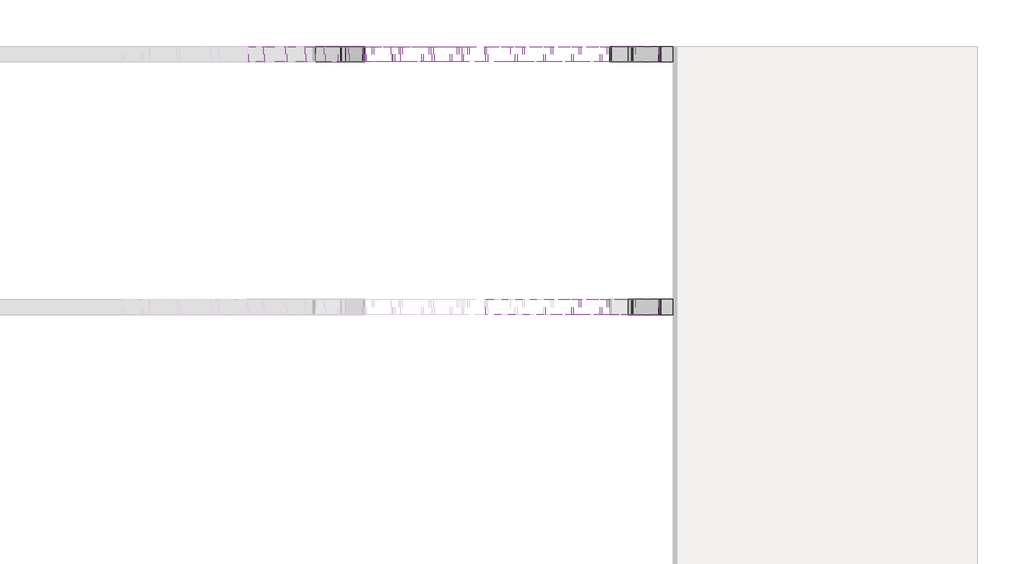
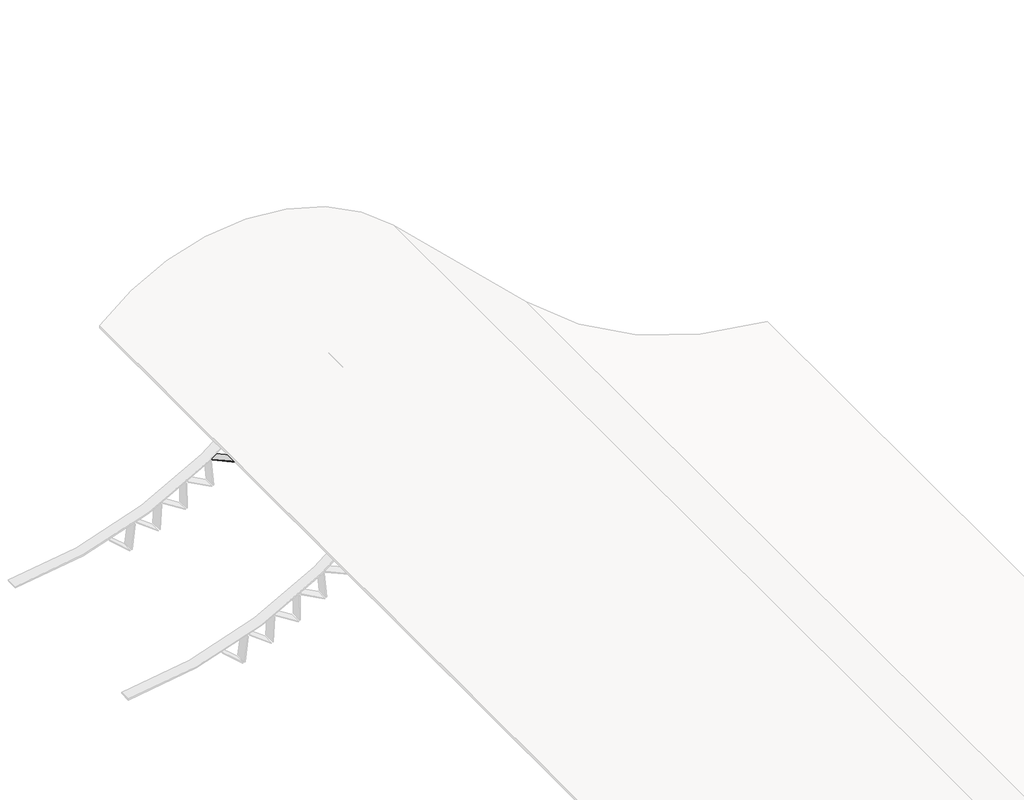
# One storey, part 16 of 16: 78 beams.
"""IFC4 building model written with IfcOpenShell, lengths in millimetres."""

import ifcopenshell
import ifcopenshell.guid

model = None  # the IFC model being written
_history = None  # IfcOwnerHistory: only IFC2X3 demands one
_inside = {}  # id of a spatial element -> (the spatial element, [elements in it])
_under = {}  # id of a project, library or spatial element -> (it, [spatial elements below it])
_declared = {}  # id of a project -> (the project, [libraries it declares])
_typed = {}  # id of a type object -> (the type object, [elements of that type])
_made_of = {}  # id of a material, layer set ... -> (it, [elements and type objects made of it])


def new_model(schema):
    """Start an empty IFC model of exactly this schema.

    Asked for "IFC4X3", IfcOpenShell would pick the latest addendum, in which some entities
    have other attributes; the version numbers below select the first issue.
    IFC2X3 requires an IfcOwnerHistory on every rooted entity: one is made here for all.
    """
    global model, _history
    if schema == "IFC4X3":
        model = ifcopenshell.file(schema_version=(4, 3, 0, 0))
    else:
        model = ifcopenshell.file(schema=schema)
    _inside.clear()
    _under.clear()
    _declared.clear()
    _typed.clear()
    _made_of.clear()
    _history = None
    if model.schema == "IFC2X3":
        org = make("IfcOrganization", Name="unknown")
        user = make(
            "IfcPersonAndOrganization",
            ThePerson=make("IfcPerson", FamilyName="unknown"),
            TheOrganization=org,
        )
        app = make(
            "IfcApplication",
            ApplicationDeveloper=org,
            Version="unknown",
            ApplicationFullName="unknown",
            ApplicationIdentifier="unknown",
        )
        _history = make(
            "IfcOwnerHistory",
            OwningUser=user,
            OwningApplication=app,
            ChangeAction="ADDED",
            CreationDate=0,
        )
    return model


def make(cls, **values):
    """One entity of the class cls with the attributes given. An attribute that is None is left unset."""
    return model.create_entity(
        cls, **{name: value for name, value in values.items() if value is not None}
    )


def rooted(cls, **values):
    """An entity with a GlobalId (a new one), such as an element, a storey or a relation."""
    return make(cls, GlobalId=ifcopenshell.guid.new(), OwnerHistory=_history, **values)


def si_unit(unit_type, name, prefix=None):
    """IfcSIUnit, for example si_unit("LENGTHUNIT", "METRE", prefix="MILLI")."""
    return make("IfcSIUnit", UnitType=unit_type, Prefix=prefix, Name=name)


def assignment(units):
    """IfcUnitAssignment: the units of a project."""
    return None if units is None else make("IfcUnitAssignment", Units=units)


def point(xyz):
    """IfcCartesianPoint."""
    return None if xyz is None else make("IfcCartesianPoint", Coordinates=xyz)


def direction(xyz):
    """IfcDirection."""
    return None if xyz is None else make("IfcDirection", DirectionRatios=xyz)


def frame(location, z_axis=None, x_axis=None):
    """IfcAxis2Placement3D, a coordinate frame: its origin and axes. An axis left out is left unset."""
    return make(
        "IfcAxis2Placement3D",
        Location=point(location),
        Axis=direction(z_axis),
        RefDirection=direction(x_axis),
    )


def frame_2d(location, x_axis=None):
    """IfcAxis2Placement2D, a coordinate frame in the plane: its origin and x axis."""
    return make(
        "IfcAxis2Placement2D", Location=point(location), RefDirection=direction(x_axis)
    )


def origin():
    """The frame at (0, 0, 0) with its axes left unset."""
    return frame((0.0, 0.0, 0.0))


def place(relative_to, where):
    """IfcLocalPlacement: puts the frame where relative to a parent placement (None: the world)."""
    return make(
        "IfcLocalPlacement", PlacementRelTo=relative_to, RelativePlacement=where
    )


def context(
    kind, dimensions, precision=None, world=None, true_north=None, identifier=None
):
    """IfcGeometricRepresentationContext, for example the 3D "Model" context."""
    return make(
        "IfcGeometricRepresentationContext",
        ContextIdentifier=identifier,
        ContextType=kind,
        CoordinateSpaceDimension=dimensions,
        Precision=precision,
        WorldCoordinateSystem=world,
        TrueNorth=true_north,
    )


def project(units=None, contexts=None):
    """IfcProject with its units and contexts."""
    return rooted(
        "IfcProject",
        Name="project",
        RepresentationContexts=contexts,
        UnitsInContext=assignment(units),
    )


def spatial(cls, under=None, at=None, **own):
    """A site, building, storey or space (cls), placed at a placement, below another one or the project."""
    s = rooted(cls, ObjectPlacement=at, **own)
    if under is not None:
        _under.setdefault(under.id(), (under, []))[1].append(s)
    return s


def polyline(points):
    """IfcPolyline through the points."""
    return make("IfcPolyline", Points=[point(p) for p in points])


def circle_curve(where, radius):
    """IfcCircle in the frame where."""
    return make("IfcCircle", Position=where, Radius=radius)


def trimmed(basis, trim1, trim2, sense, master):
    """IfcTrimmedCurve: the piece of a basis curve between two trims."""
    return make(
        "IfcTrimmedCurve",
        BasisCurve=basis,
        Trim1=trim1,
        Trim2=trim2,
        SenseAgreement=sense,
        MasterRepresentation=master,
    )


def segment(curve, same_sense, transition):
    """IfcCompositeCurveSegment."""
    return make(
        "IfcCompositeCurveSegment",
        Transition=transition,
        SameSense=same_sense,
        ParentCurve=curve,
    )


def composite_curve(segments, self_intersect=None):
    """IfcCompositeCurve: segments joined end to end."""
    return make("IfcCompositeCurve", Segments=segments, SelfIntersect=self_intersect)


def outline(outer, holes=None, kind="AREA"):
    """IfcArbitraryClosedProfileDef: a profile drawn as a closed curve; with holes, ...WithVoids."""
    if holes is None:
        return make("IfcArbitraryClosedProfileDef", ProfileType=kind, OuterCurve=outer)
    return make(
        "IfcArbitraryProfileDefWithVoids",
        ProfileType=kind,
        OuterCurve=outer,
        InnerCurves=holes,
    )


def extrude(swept, where, along, depth):
    """IfcExtrudedAreaSolid: the profile swept, set in the frame where, extruded along a direction by depth."""
    return make(
        "IfcExtrudedAreaSolid",
        SweptArea=swept,
        Position=where,
        ExtrudedDirection=direction(along),
        Depth=depth,
    )


def shape(context_of_items, identifier, shape_type, items):
    """IfcShapeRepresentation: the items that make up one representation, for example the "Body"."""
    return make(
        "IfcShapeRepresentation",
        ContextOfItems=context_of_items,
        RepresentationIdentifier=identifier,
        RepresentationType=shape_type,
        Items=items,
    )


def source(mapping_origin, context_of_items, identifier, shape_type, items):
    """IfcRepresentationMap: a shape defined once, which mapped items show again and again."""
    return make(
        "IfcRepresentationMap",
        MappingOrigin=mapping_origin,
        MappedRepresentation=shape(context_of_items, identifier, shape_type, items),
    )


def transform(
    local_origin,
    x_axis=None,
    y_axis=None,
    z_axis=None,
    scale=None,
    scale2=None,
    scale3=None,
    uniform=True,
):
    """IfcCartesianTransformationOperator3D, or its non-uniform kind. x_axis, y_axis, z_axis: its Axis1, 2, 3."""
    if uniform:
        return make(
            "IfcCartesianTransformationOperator3D",
            Axis1=direction(x_axis),
            Axis2=direction(y_axis),
            LocalOrigin=point(local_origin),
            Scale=scale,
            Axis3=direction(z_axis),
        )
    return make(
        "IfcCartesianTransformationOperator3DnonUniform",
        Axis1=direction(x_axis),
        Axis2=direction(y_axis),
        LocalOrigin=point(local_origin),
        Scale=scale,
        Axis3=direction(z_axis),
        Scale2=scale2,
        Scale3=scale3,
    )


def mapped(mapping_source, mapping_target):
    """IfcMappedItem: shows the shape of a source again, moved by a transform."""
    return make(
        "IfcMappedItem", MappingSource=mapping_source, MappingTarget=mapping_target
    )


def made_of(thing, what):
    """Note that an element or type object is made of a material, layer set ...; save() writes the relation."""
    if what is not None:
        _made_of.setdefault(what.id(), (what, []))[1].append(thing)
    return thing


def element(
    cls,
    number,
    at=None,
    inside=None,
    cuts=None,
    type_object=None,
    material=None,
    context=None,
    identifier="Body",
    shape_type=None,
    held_by="IfcProductDefinitionShape",
    body=None,
    shapes=None,
    **own,
):
    """One element of the class cls, such as IfcWall. Its Tag is "e" and its number.

    at: its placement. inside: the storey or other place that contains it. cuts: it is an
    opening in that element (IfcRelVoidsElement). A single representation is given by context,
    identifier, shape_type and body (its items); several are given by shapes. held_by: the class
    of the entity that holds the representations. save() writes the other relations.
    """
    e = rooted(cls, Tag="e%d" % number, ObjectPlacement=at, **own)
    if body is not None:
        shapes = [shape(context, identifier, shape_type, body)]
    if shapes is not None:
        e.Representation = make(held_by, Representations=shapes)
    if inside is not None:
        _inside.setdefault(inside.id(), (inside, []))[1].append(e)
    if cuts is not None:
        rooted(
            "IfcRelVoidsElement", RelatingBuildingElement=cuts, RelatedOpeningElement=e
        )
    if type_object is not None:
        _typed.setdefault(type_object.id(), (type_object, []))[1].append(e)
    return made_of(e, material)


def aggregate(whole, parts):
    """IfcRelAggregates: a whole, such as a stair, and the parts it consists of."""
    return rooted("IfcRelAggregates", RelatingObject=whole, RelatedObjects=parts)


def save(model, path):
    """Write the relations noted so far, then the file.

    IfcRelAggregates (storeys below a building ...), IfcRelContainedInSpatialStructure (elements
    in a storey), IfcRelDefinesByType, IfcRelAssociatesMaterial and IfcRelDeclares: one each for
    every whole, place, type object, material and project.
    """
    for whole, parts in _under.values():
        aggregate(whole, parts)
    for where, things in _inside.values():
        rooted(
            "IfcRelContainedInSpatialStructure",
            RelatedElements=things,
            RelatingStructure=where,
        )
    for kind, things in _typed.values():
        rooted("IfcRelDefinesByType", RelatedObjects=things, RelatingType=kind)
    for what, things in _made_of.values():
        rooted("IfcRelAssociatesMaterial", RelatedObjects=things, RelatingMaterial=what)
    for by, libraries in _declared.values():
        rooted("IfcRelDeclares", RelatingContext=by, RelatedDefinitions=libraries)
    model.write(path)


def placa_diagonal_7fe59f73(model_context):
    return source(origin(), model_context, "Body", "SweptSolid", [
        extrude(outline(polyline([(166.951958, 75.0), (166.951958, -75.0), (-167.3065458, -75.0), (-167.3065458, 75.0), (166.951958, 75.0)])), frame((0.0, 0.0, -4.0), z_axis=(0.0, 0.0, 1.0), x_axis=(1.0, 0.0, 0.0)), (0.0, 0.0, 1.0), 8.0),
    ])


def placa_diagonal_1af65b22(model_context):
    return source(origin(), model_context, "Body", "SweptSolid", [
        extrude(outline(polyline([(169.9719585, 75.0), (169.9719585, -75.0), (-169.5739238, -75.0), (-169.5739238, 75.0), (169.9719585, 75.0)])), frame((0.0, 0.0, -4.0), z_axis=(0.0, 0.0, 1.0), x_axis=(1.0, 0.0, 0.0)), (0.0, 0.0, 1.0), 8.0),
    ])


def placa_diagonal_5ef1143b(model_context):
    return source(origin(), model_context, "Body", "SweptSolid", [
        extrude(outline(polyline([(165.496273, 75.0), (165.496273, -75.0), (-165.1705217, -75.0), (-165.1705217, 75.0), (165.496273, 75.0)])), frame((0.0, 0.0, -4.0), z_axis=(0.0, 0.0, 1.0), x_axis=(1.0, 0.0, 0.0)), (0.0, 0.0, 1.0), 8.0),
    ])


def placa_diagonal_9b2e6b67(model_context):
    return source(origin(), model_context, "Body", "SweptSolid", [
        extrude(outline(polyline([(169.9719577, 75.0), (169.9719577, -75.0), (-169.573923, -75.0), (-169.573923, 75.0), (169.9719577, 75.0)])), frame((0.0, 0.0, -4.0), z_axis=(0.0, 0.0, 1.0), x_axis=(1.0, 0.0, 0.0)), (0.0, 0.0, 1.0), 8.0),
    ])


def placa_diagonal_5f8fd6b3(model_context):
    return source(origin(), model_context, "Body", "SweptSolid", [
        extrude(outline(polyline([(165.7219053, 75.0), (165.7219053, -75.0), (-165.392588, -75.0), (-165.392588, 75.0), (165.7219053, 75.0)])), frame((0.0, 0.0, -4.0), z_axis=(0.0, 0.0, 1.0), x_axis=(1.0, 0.0, 0.0)), (0.0, 0.0, 1.0), 8.0),
    ])


def placa_diagonal_668a1444(model_context):
    return source(origin(), model_context, "Body", "SweptSolid", [
        extrude(outline(polyline([(169.8505328, 75.0), (169.8505328, -75.0), (-169.6110753, -75.0), (-169.6110753, 75.0), (169.8505328, 75.0)])), frame((0.0, 0.0, -4.0), z_axis=(0.0, 0.0, 1.0), x_axis=(1.0, 0.0, 0.0)), (0.0, 0.0, 1.0), 8.0),
    ])


def placa_diagonal_fbff302d(model_context):
    return source(origin(), model_context, "Body", "SweptSolid", [
        extrude(outline(polyline([(168.0075515, 75.0), (168.0075515, -75.0), (-168.0075515, -75.0), (-168.0075515, 75.0), (168.0075515, 75.0)])), frame((0.0, 0.0, -4.0), z_axis=(0.0, 0.0, 1.0), x_axis=(1.0, 0.0, 0.0)), (0.0, 0.0, 1.0), 8.0),
    ])


def placa_diagonal_c6130ff1(model_context):
    return source(origin(), model_context, "Body", "SweptSolid", [
        extrude(outline(polyline([(169.7794224, 75.0), (169.7794224, -75.0), (-169.7794224, -75.0), (-169.7794224, 75.0), (169.7794224, 75.0)])), frame((0.0, 0.0, -4.0), z_axis=(0.0, 0.0, 1.0), x_axis=(1.0, 0.0, 0.0)), (0.0, 0.0, 1.0), 8.0),
    ])


def placa_diagonal_3ead9384(model_context):
    return source(origin(), model_context, "Body", "SweptSolid", [
        extrude(outline(polyline([(168.0075509, 75.0), (168.0075509, -75.0), (-168.0075509, -75.0), (-168.0075509, 75.0), (168.0075509, 75.0)])), frame((0.0, 0.0, -4.0), z_axis=(0.0, 0.0, 1.0), x_axis=(1.0, 0.0, 0.0)), (0.0, 0.0, 1.0), 8.0),
    ])


def placa_diagonal_77673082(model_context):
    return source(origin(), model_context, "Body", "SweptSolid", [
        extrude(outline(polyline([(164.7911476, 75.0), (164.7911476, -75.0), (-164.7911476, -75.0), (-164.7911476, 75.0), (164.7911476, 75.0)])), frame((0.0, 0.0, -4.0), z_axis=(0.0, 0.0, 1.0), x_axis=(1.0, 0.0, 0.0)), (0.0, 0.0, 1.0), 8.0),
    ])


def placa_diagonal_30fa4039(model_context):
    return source(origin(), model_context, "Body", "SweptSolid", [
        extrude(outline(polyline([(167.0675386, 75.0), (167.0675386, -75.0), (-167.4240159, -75.0), (-167.4240159, 75.0), (167.0675386, 75.0)])), frame((0.0, 0.0, -4.0), z_axis=(0.0, 0.0, 1.0), x_axis=(1.0, 0.0, 0.0)), (0.0, 0.0, 1.0), 8.0),
    ])


def placa_diagonal_ded414cc(model_context):
    return source(origin(), model_context, "Body", "SweptSolid", [
        extrude(outline(polyline([(167.4240165, 75.0), (167.4240165, -75.0), (-167.0675392, -75.0), (-167.0675392, 75.0), (167.4240165, 75.0)])), frame((0.0, 0.0, -4.0), z_axis=(0.0, 0.0, 1.0), x_axis=(1.0, 0.0, 0.0)), (0.0, 0.0, 1.0), 8.0),
    ])


def placa_diagonal_4690b74a(model_context):
    return source(origin(), model_context, "Body", "SweptSolid", [
        extrude(outline(polyline([(167.0675389, 75.0), (167.0675389, -75.0), (-167.4240162, -75.0), (-167.4240162, 75.0), (167.0675389, 75.0)])), frame((0.0, 0.0, -4.0), z_axis=(0.0, 0.0, 1.0), x_axis=(1.0, 0.0, 0.0)), (0.0, 0.0, 1.0), 8.0),
    ])


def placa_diagonal_780d3588(model_context):
    return source(origin(), model_context, "Body", "SweptSolid", [
        extrude(outline(polyline([(167.4240168, 75.0), (167.4240168, -75.0), (-167.0675395, -75.0), (-167.0675395, 75.0), (167.4240168, 75.0)])), frame((0.0, 0.0, -4.0), z_axis=(0.0, 0.0, 1.0), x_axis=(1.0, 0.0, 0.0)), (0.0, 0.0, 1.0), 8.0),
    ])


def placa_diagonal_4478edde(model_context):
    return source(origin(), model_context, "Body", "SweptSolid", [
        extrude(outline(polyline([(167.0675392, 75.0), (167.0675392, -75.0), (-167.4240165, -75.0), (-167.4240165, 75.0), (167.0675392, 75.0)])), frame((0.0, 0.0, -4.0), z_axis=(0.0, 0.0, 1.0), x_axis=(1.0, 0.0, 0.0)), (0.0, 0.0, 1.0), 8.0),
    ])


def placa_diagonal_266b1673(model_context):
    return source(origin(), model_context, "Body", "SweptSolid", [
        extrude(outline(polyline([(167.1833817, 75.0), (167.1833817, -75.0), (-167.541755, -75.0), (-167.541755, 75.0), (167.1833817, 75.0)])), frame((0.0, 0.0, -4.0), z_axis=(0.0, 0.0, 1.0), x_axis=(1.0, 0.0, 0.0)), (0.0, 0.0, 1.0), 8.0),
    ])


def placa_diagonal_df0326e2(model_context):
    return source(origin(), model_context, "Body", "SweptSolid", [
        extrude(outline(polyline([(167.0675395, 75.0), (167.0675395, -75.0), (-167.4240168, -75.0), (-167.4240168, 75.0), (167.0675395, 75.0)])), frame((0.0, 0.0, -4.0), z_axis=(0.0, 0.0, 1.0), x_axis=(1.0, 0.0, 0.0)), (0.0, 0.0, 1.0), 8.0),
    ])


def placa_diagonal_d82de291(model_context):
    return source(origin(), model_context, "Body", "SweptSolid", [
        extrude(outline(polyline([(167.0694488, 75.0), (167.0694488, -75.0), (-167.4259573, -75.0), (-167.4259573, 75.0), (167.0694488, 75.0)])), frame((0.0, 0.0, -4.0), z_axis=(0.0, 0.0, 1.0), x_axis=(1.0, 0.0, 0.0)), (0.0, 0.0, 1.0), 8.0),
    ])


def placa_diagonal_41f6052a(model_context):
    return source(origin(), model_context, "Body", "SweptSolid", [
        extrude(outline(polyline([(167.3896443, 75.0), (167.3896443, -75.0), (-167.5872499, -75.0), (-167.5872499, 75.0), (167.3896443, 75.0)])), frame((0.0, 0.0, -4.0), z_axis=(0.0, 0.0, 1.0), x_axis=(1.0, 0.0, 0.0)), (0.0, 0.0, 1.0), 8.0),
    ])


def placa_diagonal_854ad00f(model_context):
    return source(origin(), model_context, "Body", "SweptSolid", [
        extrude(outline(polyline([(168.6204795, 75.0), (168.6204795, -75.0), (-168.6204795, -75.0), (-168.6204795, 75.0), (168.6204795, 75.0)])), frame((0.0, 0.0, -4.0), z_axis=(0.0, 0.0, 1.0), x_axis=(1.0, 0.0, 0.0)), (0.0, 0.0, 1.0), 8.0),
    ])


def placa_diagonal_d8887dd5(model_context):
    return source(origin(), model_context, "Body", "SweptSolid", [
        extrude(outline(polyline([(168.6204805, 75.0), (168.6204805, -75.0), (-168.6204805, -75.0), (-168.6204805, 75.0), (168.6204805, 75.0)])), frame((0.0, 0.0, -4.0), z_axis=(0.0, 0.0, 1.0), x_axis=(1.0, 0.0, 0.0)), (0.0, 0.0, 1.0), 8.0),
    ])


def placa_diagonal_cdd87bdc(model_context):
    return source(origin(), model_context, "Body", "SweptSolid", [
        extrude(outline(polyline([(162.1535761, 75.0), (162.1535761, -75.0), (-186.2011239, -75.0), (-186.2011239, 75.0), (162.1535761, 75.0)])), frame((0.0, 0.0, -4.0), z_axis=(0.0, 0.0, 1.0), x_axis=(1.0, 0.0, 0.0)), (0.0, 0.0, 1.0), 8.0),
    ])


def placa_diagonal_28543f3d(model_context):
    return source(origin(), model_context, "Body", "SweptSolid", [
        extrude(outline(polyline([(146.2783525, 75.0), (146.2783525, -75.0), (-146.2783525, -75.0), (-146.2783525, 75.0), (146.2783525, 75.0)])), frame((0.0, 0.0, -4.0), z_axis=(0.0, 0.0, 1.0), x_axis=(1.0, 0.0, 0.0)), (0.0, 0.0, 1.0), 8.0),
    ])


def placa_diagonal_99230a8a(model_context):
    return source(origin(), model_context, "Body", "SweptSolid", [
        extrude(outline(polyline([(169.7267346, 75.0), (169.7267346, -75.0), (-168.8798643, -75.0), (-168.8798643, 75.0), (169.7267346, 75.0)])), frame((0.0, 0.0, -4.0), z_axis=(0.0, 0.0, 1.0), x_axis=(1.0, 0.0, 0.0)), (0.0, 0.0, 1.0), 8.0),
    ])


def placa_diagonal_d92fe461(model_context):
    return source(origin(), model_context, "Body", "SweptSolid", [
        extrude(outline(polyline([(171.6122376, 75.0), (171.6122376, -75.0), (-170.6977745, -75.0), (-170.6977745, 75.0), (171.6122376, 75.0)])), frame((0.0, 0.0, -4.0), z_axis=(0.0, 0.0, 1.0), x_axis=(1.0, 0.0, 0.0)), (0.0, 0.0, 1.0), 8.0),
    ])


def placa_diagonal_b60869c1(model_context):
    return source(origin(), model_context, "Body", "SweptSolid", [
        extrude(outline(polyline([(170.6977773, 75.0), (170.6977773, -75.0), (-171.6122404, -75.0), (-171.6122404, 75.0), (170.6977773, 75.0)])), frame((0.0, 0.0, -4.0), z_axis=(0.0, 0.0, 1.0), x_axis=(1.0, 0.0, 0.0)), (0.0, 0.0, 1.0), 8.0),
    ])


def placa_diagonal_c1c8cf8f(model_context):
    return source(origin(), model_context, "Body", "SweptSolid", [
        extrude(outline(polyline([(171.6122393, 75.0), (171.6122393, -75.0), (-170.6977761, -75.0), (-170.6977761, 75.0), (171.6122393, 75.0)])), frame((0.0, 0.0, -4.0), z_axis=(0.0, 0.0, 1.0), x_axis=(1.0, 0.0, 0.0)), (0.0, 0.0, 1.0), 8.0),
    ])


def placa_diagonal_c2f8bddd(model_context):
    return source(origin(), model_context, "Body", "SweptSolid", [
        extrude(outline(polyline([(170.6977754, 75.0), (170.6977754, -75.0), (-171.6122385, -75.0), (-171.6122385, 75.0), (170.6977754, 75.0)])), frame((0.0, 0.0, -4.0), z_axis=(0.0, 0.0, 1.0), x_axis=(1.0, 0.0, 0.0)), (0.0, 0.0, 1.0), 8.0),
    ])


def placa_diagonal_cac56629(model_context):
    return source(origin(), model_context, "Body", "SweptSolid", [
        extrude(outline(polyline([(171.6122413, 75.0), (171.6122413, -75.0), (-170.6977781, -75.0), (-170.6977781, 75.0), (171.6122413, 75.0)])), frame((0.0, 0.0, -4.0), z_axis=(0.0, 0.0, 1.0), x_axis=(1.0, 0.0, 0.0)), (0.0, 0.0, 1.0), 8.0),
    ])


def placa_diagonal_d971223c(model_context):
    return source(origin(), model_context, "Body", "SweptSolid", [
        extrude(outline(polyline([(170.6977735, 75.0), (170.6977735, -75.0), (-171.6122365, -75.0), (-171.6122365, 75.0), (170.6977735, 75.0)])), frame((0.0, 0.0, -4.0), z_axis=(0.0, 0.0, 1.0), x_axis=(1.0, 0.0, 0.0)), (0.0, 0.0, 1.0), 8.0),
    ])


def placa_diagonal_acf5f4f6(model_context):
    return source(origin(), model_context, "Body", "SweptSolid", [
        extrude(outline(polyline([(171.6122387, 75.0), (171.6122387, -75.0), (-170.6977756, -75.0), (-170.6977756, 75.0), (171.6122387, 75.0)])), frame((0.0, 0.0, -4.0), z_axis=(0.0, 0.0, 1.0), x_axis=(1.0, 0.0, 0.0)), (0.0, 0.0, 1.0), 8.0),
    ])


def placa_diagonal_348c000d(model_context):
    return source(origin(), model_context, "Body", "SweptSolid", [
        extrude(outline(polyline([(169.5917652, 75.0), (169.5917652, -75.0), (-170.4649339, -75.0), (-170.4649339, 75.0), (169.5917652, 75.0)])), frame((0.0, 0.0, -4.0), z_axis=(0.0, 0.0, 1.0), x_axis=(1.0, 0.0, 0.0)), (0.0, 0.0, 1.0), 8.0),
    ])


def placa_diagonal_616b5fb7(model_context):
    return source(origin(), model_context, "Body", "SweptSolid", [
        extrude(outline(polyline([(172.7806227, 75.0), (172.7806227, -75.0), (-171.8235671, -75.0), (-171.8235671, 75.0), (172.7806227, 75.0)])), frame((0.0, 0.0, -4.0), z_axis=(0.0, 0.0, 1.0), x_axis=(1.0, 0.0, 0.0)), (0.0, 0.0, 1.0), 8.0),
    ])


def placa_diagonal_a2e3544b(model_context):
    return source(origin(), model_context, "Body", "SweptSolid", [
        extrude(outline(polyline([(165.536904, 75.0), (165.536904, -75.0), (-166.2630935, -75.0), (-166.2630935, 75.0), (165.536904, 75.0)])), frame((0.0, 0.0, -4.0), z_axis=(0.0, 0.0, 1.0), x_axis=(1.0, 0.0, 0.0)), (0.0, 0.0, 1.0), 8.0),
    ])


def placa_diagonal_9cc04f9e(model_context):
    return source(origin(), model_context, "Body", "SweptSolid", [
        extrude(outline(polyline([(177.4551585, 75.0), (177.4551585, -75.0), (-176.322012, -75.0), (-176.322012, 75.0), (177.4551585, 75.0)])), frame((0.0, 0.0, -4.0), z_axis=(0.0, 0.0, 1.0), x_axis=(1.0, 0.0, 0.0)), (0.0, 0.0, 1.0), 8.0),
    ])


def placa_diagonal_a33581f3(model_context):
    return source(origin(), model_context, "Body", "SweptSolid", [
        extrude(outline(polyline([(146.2839954, 75.0), (146.2839954, -75.0), (-146.2743867, -75.0), (-146.2743867, 75.0), (146.2839954, 75.0)])), frame((0.0, 0.0, -4.0), z_axis=(0.0, 0.0, 1.0), x_axis=(1.0, 0.0, 0.0)), (0.0, 0.0, 1.0), 8.0),
    ])


model = new_model("IFC4")

# Units and contexts
model_context = context("Model", 3, world=origin())
ifc_project = project(units=[si_unit("LENGTHUNIT", "METRE", prefix="MILLI")], contexts=[model_context])

# Site, building, storey
site = spatial("IfcSite", under=ifc_project)
building = spatial("IfcBuilding", under=site)
storey = spatial("IfcBuildingStorey", under=building, Name="Nível 5", Elevation=48665.0)

# Beams
placement = place(None, origin())
element("IfcBeam", 1, ObjectType="Placa : banzo", at=placement, inside=storey, context=model_context, shape_type="SweptSolid", body=[
    extrude(outline(polyline([(0.0, -150.0), (0.0, 0.0), (2344.6326009, 0.0), (2344.6326009, -150.0), (0.0, -150.0)])), frame((4748.0759643, 15321.4376366, 49634.6077), z_axis=(0.6913289930670965, 0.0, 0.7225401188479672), x_axis=(-0.7225401188479672, 0.0, 0.6913289930670965)), (0.0, 0.0, 1.0), 16.0),
])
element("IfcBeam", 2, ObjectType="Placa : banzo", at=placement, inside=storey, context=model_context, shape_type="SweptSolid", body=[
    extrude(outline(polyline([(0.0, -150.0), (0.0, 0.0), (2017.4057636, 0.0), (2017.4057636, -150.0), (0.0, -150.0)])), frame((3301.480628, 15321.4376366, 51029.2987951), z_axis=(-0.6913289930670814, 0.0, 0.7225401188479816), x_axis=(-0.7225401188479816, 0.0, -0.6913289930670814)), (0.0, 0.0, 1.0), 16.0),
])
element("IfcBeam", 3, ObjectType="Placa : banzo", at=placement, inside=storey, context=model_context, shape_type="SweptSolid", body=[
    extrude(outline(polyline([(0.0, -150.0), (0.0, 0.0), (1981.537589, 0.0), (1981.537589, -150.0), (0.0, -150.0)])), frame((3044.6605493, 15321.4376366, 51245.8304858), z_axis=(-0.6913289930670827, 0.0, 0.7225401188479804), x_axis=(-0.7225401188479804, 0.0, -0.6913289930670827)), (0.0, 0.0, 1.0), 16.0),
])
element("IfcBeam", 4, ObjectType="Placa : banzo", at=placement, inside=storey, context=model_context, shape_type="SweptSolid", body=[
    extrude(outline(composite_curve([segment(polyline([(48491.8888252, 8136.0015515), (48507.8570745, 8137.0090317)]), True, "CONTINUOUS"), segment(trimmed(circle_curve(frame_2d((53506.1312788, 8452.3636953)), 5008.2126139), [point((48507.8570745, 8137.0090317))], [point((49887.4967416, 4990.0411119))], True, "CARTESIAN"), True, "CONTINUOUS"), segment(polyline([(49887.4967416, 4990.0411119), (49875.9360997, 4978.979848)]), True, "CONTINUOUS"), segment(trimmed(circle_curve(frame_2d((53506.1312788, 8452.3636953)), 5024.2126139), [point((49875.9360997, 4978.979848))], [point((48491.8888252, 8136.0015515))], False, "CARTESIAN"), True, "CONTINUOUS")], self_intersect=False)), frame((0.0, 15321.4376366, 0.0), z_axis=(0.0, 1.0, 0.0), x_axis=(0.0, 0.0, 1.0)), (0.0, 0.0, 1.0), 150.0),
])
element("IfcBeam", 5, ObjectType="Placa : banzo", at=placement, inside=storey, context=model_context, shape_type="SweptSolid", body=[
    extrude(outline(polyline([(0.0, -150.0), (0.0, 0.0), (2344.6326009, 0.0), (2344.6326009, -150.0), (0.0, -150.0)])), frame((4978.979848, 15321.4376366, 49875.9360997), z_axis=(0.6913289930670943, 0.0, 0.7225401188479692), x_axis=(-0.7225401188479692, 0.0, 0.6913289930670943)), (0.0, 0.0, 1.0), 16.0),
])
element("IfcBeam", 6, ObjectType="Placa : banzo", at=placement, inside=storey, context=model_context, shape_type="SweptSolid", body=[
    extrude(outline(composite_curve([segment(polyline([(48491.8888252, 8136.0015515), (48507.8570745, 8137.0090317)]), True, "CONTINUOUS"), segment(trimmed(circle_curve(frame_2d((53506.1312788, 8452.3636953)), 5008.2126139), [point((48507.8570745, 8137.0090317))], [point((49887.4967416, 4990.0411119))], True, "CARTESIAN"), True, "CONTINUOUS"), segment(polyline([(49887.4967416, 4990.0411119), (49875.9360997, 4978.979848)]), True, "CONTINUOUS"), segment(trimmed(circle_curve(frame_2d((53506.1312788, 8452.3636953)), 5024.2126139), [point((49875.9360997, 4978.979848))], [point((48491.8888252, 8136.0015515))], False, "CARTESIAN"), True, "CONTINUOUS")], self_intersect=False)), frame((0.0, 12821.4376366, 0.0), z_axis=(0.0, 1.0, 0.0), x_axis=(0.0, 0.0, 1.0)), (0.0, 0.0, 1.0), 150.0),
])
element("IfcBeam", 7, ObjectType="Placa : banzo", at=placement, inside=storey, context=model_context, shape_type="SweptSolid", body=[
    extrude(outline(polyline([(0.0, -150.0), (0.0, 0.0), (2344.6326009, 0.0), (2344.6326009, -150.0), (0.0, -150.0)])), frame((4978.979848, 12821.4376366, 49875.9360997), z_axis=(0.6913289930670943, 0.0, 0.7225401188479692), x_axis=(-0.7225401188479692, 0.0, 0.6913289930670943)), (0.0, 0.0, 1.0), 16.0),
])
placa_diagonal_shape = placa_diagonal_7fe59f73(model_context)
element("IfcBeam", 8, ObjectType="Placa : diagonal", at=placement, inside=storey, context=model_context, shape_type="MappedRepresentation", body=[
    mapped(placa_diagonal_shape, transform((5928.9944426, 15396.4376366, 48979.584917), x_axis=(0.0, 0.0, 1.0), y_axis=(0.0, -1.0, 0.0), z_axis=(1.0, 0.0, 0.0))),
])
element("IfcBeam", 9, ObjectType="Placa : diagonal", at=placement, inside=storey, context=model_context, shape_type="MappedRepresentation", body=[
    mapped(placa_diagonal_shape, transform((5928.9944426, 12896.4376366, 48979.584917), x_axis=(0.0, 0.0, 1.0), y_axis=(0.0, -1.0, 0.0), z_axis=(1.0, 0.0, 0.0))),
])
placa_diagonal_2_shape = placa_diagonal_1af65b22(model_context)
element("IfcBeam", 10, ObjectType="Placa : diagonal", at=placement, inside=storey, context=model_context, shape_type="MappedRepresentation", body=[
    mapped(placa_diagonal_2_shape, transform((1129.4090602, 15396.4376366, 49273.3369453), x_axis=(0.9127247118647549, 0.0, -0.4085750853287561), y_axis=(0.0, -1.0, 0.0), z_axis=(-0.4085750853287561, 0.0, -0.9127247118647549))),
])
placa_diagonal_3_shape = placa_diagonal_5ef1143b(model_context)
element("IfcBeam", 11, ObjectType="Placa : diagonal", at=placement, inside=storey, context=model_context, shape_type="MappedRepresentation", body=[
    mapped(placa_diagonal_3_shape, transform((1276.3296406, 15396.4376366, 49380.807103), x_axis=(0.16004805378550413, 0.0, -0.9871092241892345), y_axis=(0.0, -1.0, 0.0), z_axis=(-0.9871092241892345, 0.0, -0.16004805378550413))),
])
placa_diagonal_4_shape = placa_diagonal_9b2e6b67(model_context)
element("IfcBeam", 12, ObjectType="Placa : diagonal", at=placement, inside=storey, context=model_context, shape_type="MappedRepresentation", body=[
    mapped(placa_diagonal_4_shape, transform((1428.5369528, 15396.4376366, 49501.3389376), x_axis=(0.9399545796535577, 0.0, -0.3412995578495579), y_axis=(0.0, -1.0, 0.0), z_axis=(-0.3412995578495579, 0.0, -0.9399545796535577))),
])
placa_diagonal_5_shape = placa_diagonal_5f8fd6b3(model_context)
element("IfcBeam", 13, ObjectType="Placa : diagonal", at=placement, inside=storey, context=model_context, shape_type="MappedRepresentation", body=[
    mapped(placa_diagonal_5_shape, transform((1567.652562, 15396.4376366, 49619.5264857), x_axis=(0.22892966378492483, 0.0, -0.9734429665056507), y_axis=(0.0, -1.0, 0.0), z_axis=(-0.9734429665056507, 0.0, -0.22892966378492483))),
])
placa_diagonal_6_shape = placa_diagonal_668a1444(model_context)
element("IfcBeam", 14, ObjectType="Placa : diagonal", at=placement, inside=storey, context=model_context, shape_type="MappedRepresentation", body=[
    mapped(placa_diagonal_6_shape, transform((1710.9295552, 15396.4376366, 49750.5482189), x_axis=(0.9613882153955893, 0.0, -0.27519574723909573), y_axis=(0.0, -1.0, 0.0), z_axis=(-0.27519574723909573, 0.0, -0.9613882153955893))),
])
placa_diagonal_7_shape = placa_diagonal_fbff302d(model_context)
element("IfcBeam", 15, ObjectType="Placa : diagonal", at=placement, inside=storey, context=model_context, shape_type="MappedRepresentation", body=[
    mapped(placa_diagonal_7_shape, transform((1850.8659492, 15396.4376366, 49883.5465197), x_axis=(0.24308407350904415, 0.0, -0.9700052232881273), y_axis=(0.0, -1.0, 0.0), z_axis=(-0.9700052232881273, 0.0, -0.24308407350904415))),
])
element("IfcBeam", 16, ObjectType="Placa : diagonal", at=placement, inside=storey, context=model_context, shape_type="MappedRepresentation", body=[
    mapped(placa_diagonal_7_shape, transform((2411.9963184, 15396.4376366, 50420.4380818), x_axis=(0.24308407331774187, 0.0, -0.9700052233360678), y_axis=(0.0, -1.0, 0.0), z_axis=(-0.9700052233360678, 0.0, -0.24308407331774187))),
])
element("IfcBeam", 17, ObjectType="Placa : diagonal", at=placement, inside=storey, context=model_context, shape_type="MappedRepresentation", body=[
    mapped(placa_diagonal_7_shape, transform((2692.5615038, 15396.4376366, 50688.8838637), x_axis=(0.24308407350903813, 0.0, -0.9700052232881288), y_axis=(0.0, -1.0, 0.0), z_axis=(-0.9700052232881288, 0.0, -0.24308407350903813))),
])
placa_diagonal_8_shape = placa_diagonal_c6130ff1(model_context)
element("IfcBeam", 18, ObjectType="Placa : diagonal", at=placement, inside=storey, context=model_context, shape_type="MappedRepresentation", body=[
    mapped(placa_diagonal_8_shape, transform((1991.148542, 15396.4376366, 50017.7694107), x_axis=(0.9631713478731971, 0.0, -0.2688883683540974), y_axis=(0.0, -1.0, 0.0), z_axis=(-0.2688883683540974, 0.0, -0.9631713478731971))),
])
element("IfcBeam", 19, ObjectType="Placa : diagonal", at=placement, inside=storey, context=model_context, shape_type="MappedRepresentation", body=[
    mapped(placa_diagonal_8_shape, transform((2271.7137256, 15396.4376366, 50286.2151908), x_axis=(0.9631713478975275, 0.0, -0.2688883682669448), y_axis=(0.0, -1.0, 0.0), z_axis=(-0.2688883682669448, 0.0, -0.9631713478975275))),
])
element("IfcBeam", 20, ObjectType="Placa : diagonal", at=placement, inside=storey, context=model_context, shape_type="MappedRepresentation", body=[
    mapped(placa_diagonal_8_shape, transform((2552.2789111, 15396.4376366, 50554.6609728), x_axis=(0.9631713478212401, 0.0, -0.2688883685402097), y_axis=(0.0, -1.0, 0.0), z_axis=(-0.2688883685402097, 0.0, -0.9631713478212401))),
])
element("IfcBeam", 21, ObjectType="Placa : diagonal", at=placement, inside=storey, context=model_context, shape_type="MappedRepresentation", body=[
    mapped(placa_diagonal_8_shape, transform((2832.8440965, 15396.4376366, 50823.1067546), x_axis=(0.96317134786801, 0.0, -0.26888836837267793), y_axis=(0.0, -1.0, 0.0), z_axis=(-0.26888836837267793, 0.0, -0.96317134786801))),
])
element("IfcBeam", 22, ObjectType="Placa : diagonal", at=placement, inside=storey, context=model_context, shape_type="MappedRepresentation", body=[
    mapped(placa_diagonal_8_shape, transform((2975.9434558, 15396.4376366, 50960.0247379), x_axis=(0.22612317814304966, 0.0, -0.9740987158940754), y_axis=(0.0, -1.0, 0.0), z_axis=(-0.9740987158940754, 0.0, -0.22612317814304966))),
])
placa_diagonal_9_shape = placa_diagonal_3ead9384(model_context)
element("IfcBeam", 23, ObjectType="Placa : diagonal", at=placement, inside=storey, context=model_context, shape_type="MappedRepresentation", body=[
    mapped(placa_diagonal_9_shape, transform((2131.4311338, 15396.4376366, 50151.9923007), x_axis=(0.24308407925127004, 0.0, -0.970005221849121), y_axis=(0.0, -1.0, 0.0), z_axis=(-0.970005221849121, 0.0, -0.24308407925127004))),
])
placa_diagonal_10_shape = placa_diagonal_77673082(model_context)
element("IfcBeam", 24, ObjectType="Placa : diagonal", at=placement, inside=storey, context=model_context, shape_type="MappedRepresentation", body=[
    mapped(placa_diagonal_10_shape, transform((3110.8606023, 15396.4376366, 51089.1139506), x_axis=(0.9480011799588844, 0.0, -0.318266810705362), y_axis=(0.0, -1.0, 0.0), z_axis=(-0.318266810705362, 0.0, -0.9480011799588844))),
])
placa_diagonal_11_shape = placa_diagonal_30fa4039(model_context)
element("IfcBeam", 25, ObjectType="Placa : diagonal", at=placement, inside=storey, context=model_context, shape_type="MappedRepresentation", body=[
    mapped(placa_diagonal_11_shape, transform((6426.8268937, 15396.4376366, 48735.9986151), x_axis=(0.7903109338244996, 0.0, 0.612705988119463), y_axis=(0.0, -1.0, 0.0), z_axis=(0.612705988119463, 0.0, -0.7903109338244996))),
])
element("IfcBeam", 26, ObjectType="Placa : diagonal", at=placement, inside=storey, context=model_context, shape_type="MappedRepresentation", body=[
    mapped(placa_diagonal_11_shape, transform((5609.0896822, 15396.4376366, 49173.3772061), x_axis=(0.07092138152000912, 0.0, 0.9974819084290669), y_axis=(0.0, -1.0, 0.0), z_axis=(0.9974819084290669, 0.0, -0.07092138152000912))),
])
element("IfcBeam", 27, ObjectType="Placa : diagonal", at=placement, inside=storey, context=model_context, shape_type="MappedRepresentation", body=[
    mapped(placa_diagonal_11_shape, transform((5304.1964204, 15396.4376366, 49389.5783795), x_axis=(0.14263158168504164, 0.0, 0.9897758493244939), y_axis=(0.0, -1.0, 0.0), z_axis=(0.9897758493244939, 0.0, -0.14263158168504164))),
])
element("IfcBeam", 28, ObjectType="Placa : diagonal", at=placement, inside=storey, context=model_context, shape_type="MappedRepresentation", body=[
    mapped(placa_diagonal_11_shape, transform((6426.8268937, 12896.4376366, 48735.9986151), x_axis=(0.7903109338244996, 0.0, 0.612705988119463), y_axis=(0.0, -1.0, 0.0), z_axis=(0.612705988119463, 0.0, -0.7903109338244996))),
])
element("IfcBeam", 29, ObjectType="Placa : diagonal", at=placement, inside=storey, context=model_context, shape_type="MappedRepresentation", body=[
    mapped(placa_diagonal_11_shape, transform((5609.0896822, 12896.4376366, 49173.3772061), x_axis=(0.07092138152000912, 0.0, 0.9974819084290669), y_axis=(0.0, -1.0, 0.0), z_axis=(0.9974819084290669, 0.0, -0.07092138152000912))),
])
element("IfcBeam", 30, ObjectType="Placa : diagonal", at=placement, inside=storey, context=model_context, shape_type="MappedRepresentation", body=[
    mapped(placa_diagonal_11_shape, transform((5304.1964204, 12896.4376366, 49389.5783795), x_axis=(0.14263158168504164, 0.0, 0.9897758493244939), y_axis=(0.0, -1.0, 0.0), z_axis=(0.9897758493244939, 0.0, -0.14263158168504164))),
])
placa_diagonal_12_shape = placa_diagonal_ded414cc(model_context)
element("IfcBeam", 31, ObjectType="Placa : diagonal", at=placement, inside=storey, context=model_context, shape_type="MappedRepresentation", body=[
    mapped(placa_diagonal_12_shape, transform((6261.5831805, 15396.4376366, 48809.59578), x_axis=(0.07323083091157225, 0.0, -0.9973150181382013), y_axis=(0.0, -1.0, 0.0), z_axis=(-0.9973150181382013, 0.0, -0.07323083091157225))),
])
element("IfcBeam", 32, ObjectType="Placa : diagonal", at=placement, inside=storey, context=model_context, shape_type="MappedRepresentation", body=[
    mapped(placa_diagonal_12_shape, transform((6261.5831805, 12896.4376366, 48809.59578), x_axis=(0.07323083091157225, 0.0, -0.9973150181382013), y_axis=(0.0, -1.0, 0.0), z_axis=(-0.9973150181382013, 0.0, -0.07323083091157225))),
])
placa_diagonal_13_shape = placa_diagonal_4690b74a(model_context)
element("IfcBeam", 33, ObjectType="Placa : diagonal", at=placement, inside=storey, context=model_context, shape_type="MappedRepresentation", body=[
    mapped(placa_diagonal_13_shape, transform((6775.9078558, 15396.4376366, 48602.4122028), x_axis=(0.7440939511464111, 0.0, 0.668074989703493), y_axis=(0.0, -1.0, 0.0), z_axis=(0.668074989703493, 0.0, -0.7440939511464111))),
])
element("IfcBeam", 34, ObjectType="Placa : diagonal", at=placement, inside=storey, context=model_context, shape_type="MappedRepresentation", body=[
    mapped(placa_diagonal_13_shape, transform((6775.9078558, 12896.4376366, 48602.4122028), x_axis=(0.7440939511464111, 0.0, 0.668074989703493), y_axis=(0.0, -1.0, 0.0), z_axis=(0.668074989703493, 0.0, -0.7440939511464111))),
])
placa_diagonal_14_shape = placa_diagonal_780d3588(model_context)
element("IfcBeam", 35, ObjectType="Placa : diagonal", at=placement, inside=storey, context=model_context, shape_type="MappedRepresentation", body=[
    mapped(placa_diagonal_14_shape, transform((6605.7893181, 15396.4376366, 48663.9078192), x_axis=(0.14492299862526645, 0.0, -0.9894429364392173), y_axis=(0.0, -1.0, 0.0), z_axis=(-0.9894429364392173, 0.0, -0.14492299862526645))),
])
element("IfcBeam", 36, ObjectType="Placa : diagonal", at=placement, inside=storey, context=model_context, shape_type="MappedRepresentation", body=[
    mapped(placa_diagonal_14_shape, transform((6605.7893181, 12896.4376366, 48663.9078192), x_axis=(0.14492299862526645, 0.0, -0.9894429364392173), y_axis=(0.0, -1.0, 0.0), z_axis=(-0.9894429364392173, 0.0, -0.14492299862526645))),
])
placa_diagonal_15_shape = placa_diagonal_4478edde(model_context)
element("IfcBeam", 37, ObjectType="Placa : diagonal", at=placement, inside=storey, context=model_context, shape_type="MappedRepresentation", body=[
    mapped(placa_diagonal_15_shape, transform((6088.2822399, 15396.4376366, 48894.3979999), x_axis=(0.8324169335826528, 0.0, 0.5541498431695647), y_axis=(0.0, -1.0, 0.0), z_axis=(0.5541498431695647, 0.0, -0.8324169335826528))),
])
element("IfcBeam", 38, ObjectType="Placa : diagonal", at=placement, inside=storey, context=model_context, shape_type="MappedRepresentation", body=[
    mapped(placa_diagonal_15_shape, transform((5153.1476633, 15396.4376366, 49509.6154791), x_axis=(0.9319923819939867, 0.0, 0.3624778612621392), y_axis=(0.0, -1.0, 0.0), z_axis=(0.3624778612621392, 0.0, -0.9319923819939867))),
])
element("IfcBeam", 39, ObjectType="Placa : diagonal", at=placement, inside=storey, context=model_context, shape_type="MappedRepresentation", body=[
    mapped(placa_diagonal_15_shape, transform((6088.2822399, 12896.4376366, 48894.3979999), x_axis=(0.8324169335826528, 0.0, 0.5541498431695647), y_axis=(0.0, -1.0, 0.0), z_axis=(0.5541498431695647, 0.0, -0.8324169335826528))),
])
element("IfcBeam", 40, ObjectType="Placa : diagonal", at=placement, inside=storey, context=model_context, shape_type="MappedRepresentation", body=[
    mapped(placa_diagonal_15_shape, transform((5153.1476633, 12896.4376366, 49509.6154791), x_axis=(0.9319923819939867, 0.0, 0.3624778612621392), y_axis=(0.0, -1.0, 0.0), z_axis=(0.3624778612621392, 0.0, -0.9319923819939867))),
])
placa_diagonal_16_shape = placa_diagonal_266b1673(model_context)
element("IfcBeam", 41, ObjectType="Placa : diagonal", at=placement, inside=storey, context=model_context, shape_type="MappedRepresentation", body=[
    mapped(placa_diagonal_16_shape, transform((5762.256454, 15396.4376366, 49076.6574425), x_axis=(0.8707619569809124, 0.0, 0.4917048039980612), y_axis=(0.0, -1.0, 0.0), z_axis=(0.4917048039980612, 0.0, -0.8707619569809124))),
])
element("IfcBeam", 42, ObjectType="Placa : diagonal", at=placement, inside=storey, context=model_context, shape_type="MappedRepresentation", body=[
    mapped(placa_diagonal_16_shape, transform((5762.256454, 12896.4376366, 49076.6574425), x_axis=(0.8707619569809124, 0.0, 0.4917048039980612), y_axis=(0.0, -1.0, 0.0), z_axis=(0.4917048039980612, 0.0, -0.8707619569809124))),
])
placa_diagonal_17_shape = placa_diagonal_df0326e2(model_context)
element("IfcBeam", 43, ObjectType="Placa : diagonal", at=placement, inside=storey, context=model_context, shape_type="MappedRepresentation", body=[
    mapped(placa_diagonal_17_shape, transform((5449.7819704, 15396.4376366, 49282.2150918), x_axis=(0.9034423838459107, 0.0, 0.42870952761843073), y_axis=(0.0, -1.0, 0.0), z_axis=(0.42870952761843073, 0.0, -0.9034423838459107))),
])
element("IfcBeam", 44, ObjectType="Placa : diagonal", at=placement, inside=storey, context=model_context, shape_type="MappedRepresentation", body=[
    mapped(placa_diagonal_17_shape, transform((5449.7819704, 12896.4376366, 49282.2150918), x_axis=(0.9034423838459107, 0.0, 0.42870952761843073), y_axis=(0.0, -1.0, 0.0), z_axis=(0.42870952761843073, 0.0, -0.9034423838459107))),
])
placa_diagonal_18_shape = placa_diagonal_d82de291(model_context)
element("IfcBeam", 45, ObjectType="Placa : diagonal", at=placement, inside=storey, context=model_context, shape_type="MappedRepresentation", body=[
    mapped(placa_diagonal_18_shape, transform((5015.6759809, 15396.4376366, 49627.1956386), x_axis=(0.21358119550637292, 0.0, 0.9769253159408188), y_axis=(0.0, -1.0, 0.0), z_axis=(0.9769253159408188, 0.0, -0.21358119550637292))),
])
element("IfcBeam", 46, ObjectType="Placa : diagonal", at=placement, inside=storey, context=model_context, shape_type="MappedRepresentation", body=[
    mapped(placa_diagonal_18_shape, transform((5015.6759809, 12896.4376366, 49627.1956386), x_axis=(0.21358119550637292, 0.0, 0.9769253159408188), y_axis=(0.0, -1.0, 0.0), z_axis=(0.9769253159408188, 0.0, -0.21358119550637292))),
])
placa_diagonal_19_shape = placa_diagonal_41f6052a(model_context)
element("IfcBeam", 47, ObjectType="Placa : diagonal", at=placement, inside=storey, context=model_context, shape_type="MappedRepresentation", body=[
    mapped(placa_diagonal_19_shape, transform((4873.422487, 15396.4376366, 49757.5497161), x_axis=(0.9554227005684277, 0.0, 0.29524136437588255), y_axis=(0.0, -1.0, 0.0), z_axis=(0.29524136437588255, 0.0, -0.9554227005684277))),
])
element("IfcBeam", 48, ObjectType="Placa : diagonal", at=placement, inside=storey, context=model_context, shape_type="MappedRepresentation", body=[
    mapped(placa_diagonal_19_shape, transform((4873.422487, 12896.4376366, 49757.5497161), x_axis=(0.9554227005684277, 0.0, 0.29524136437588255), y_axis=(0.0, -1.0, 0.0), z_axis=(0.29524136437588255, 0.0, -0.9554227005684277))),
])
placa_diagonal_20_shape = placa_diagonal_854ad00f(model_context)
element("IfcBeam", 49, ObjectType="Placa : diagonal", at=placement, inside=storey, context=model_context, shape_type="MappedRepresentation", body=[
    mapped(placa_diagonal_20_shape, transform((4736.0330553, 15396.4376366, 49888.3314828), x_axis=(0.2371249830724848, 0.0, 0.971479151810719), y_axis=(0.0, -1.0, 0.0), z_axis=(0.971479151810719, 0.0, -0.2371249830724848))),
])
element("IfcBeam", 50, ObjectType="Placa : diagonal", at=placement, inside=storey, context=model_context, shape_type="MappedRepresentation", body=[
    mapped(placa_diagonal_20_shape, transform((4457.1633463, 15396.4376366, 50155.1550267), x_axis=(0.23712498292118317, 0.0, 0.9714791518476495), y_axis=(0.0, -1.0, 0.0), z_axis=(0.9714791518476495, 0.0, -0.23712498292118317))),
])
element("IfcBeam", 51, ObjectType="Placa : diagonal", at=placement, inside=storey, context=model_context, shape_type="MappedRepresentation", body=[
    mapped(placa_diagonal_20_shape, transform((4178.2936373, 15396.4376366, 50421.9785706), x_axis=(0.2371249830724861, 0.0, 0.9714791518107186), y_axis=(0.0, -1.0, 0.0), z_axis=(0.9714791518107186, 0.0, -0.2371249830724861))),
])
element("IfcBeam", 52, ObjectType="Placa : diagonal", at=placement, inside=storey, context=model_context, shape_type="MappedRepresentation", body=[
    mapped(placa_diagonal_20_shape, transform((3899.4239283, 15396.4376366, 50688.8021133), x_axis=(0.23712498292776307, 0.0, 0.9714791518460436), y_axis=(0.0, -1.0, 0.0), z_axis=(0.9714791518460436, 0.0, -0.23712498292776307))),
])
element("IfcBeam", 53, ObjectType="Placa : diagonal", at=placement, inside=storey, context=model_context, shape_type="MappedRepresentation", body=[
    mapped(placa_diagonal_20_shape, transform((3620.5542193, 15396.4376366, 50955.6256565), x_axis=(0.23712498292776307, 0.0, 0.9714791518460436), y_axis=(0.0, -1.0, 0.0), z_axis=(0.9714791518460436, 0.0, -0.23712498292776307))),
])
element("IfcBeam", 54, ObjectType="Placa : diagonal", at=placement, inside=storey, context=model_context, shape_type="MappedRepresentation", body=[
    mapped(placa_diagonal_20_shape, transform((4736.0330553, 12896.4376366, 49888.3314828), x_axis=(0.2371249830724848, 0.0, 0.971479151810719), y_axis=(0.0, -1.0, 0.0), z_axis=(0.971479151810719, 0.0, -0.2371249830724848))),
])
element("IfcBeam", 55, ObjectType="Placa : diagonal", at=placement, inside=storey, context=model_context, shape_type="MappedRepresentation", body=[
    mapped(placa_diagonal_20_shape, transform((4457.1633463, 12896.4376366, 50155.1550267), x_axis=(0.23712498292118317, 0.0, 0.9714791518476495), y_axis=(0.0, -1.0, 0.0), z_axis=(0.9714791518476495, 0.0, -0.23712498292118317))),
])
element("IfcBeam", 56, ObjectType="Placa : diagonal", at=placement, inside=storey, context=model_context, shape_type="MappedRepresentation", body=[
    mapped(placa_diagonal_20_shape, transform((4178.2936373, 12896.4376366, 50421.9785706), x_axis=(0.2371249830724861, 0.0, 0.9714791518107186), y_axis=(0.0, -1.0, 0.0), z_axis=(0.9714791518107186, 0.0, -0.2371249830724861))),
])
placa_diagonal_21_shape = placa_diagonal_d8887dd5(model_context)
element("IfcBeam", 57, ObjectType="Placa : diagonal", at=placement, inside=storey, context=model_context, shape_type="MappedRepresentation", body=[
    mapped(placa_diagonal_21_shape, transform((4596.5982008, 15396.4376366, 50021.7432547), x_axis=(0.96006884625819, 0.0, 0.2797638476366589), y_axis=(0.0, -1.0, 0.0), z_axis=(0.2797638476366589, 0.0, -0.96006884625819))),
])
element("IfcBeam", 58, ObjectType="Placa : diagonal", at=placement, inside=storey, context=model_context, shape_type="MappedRepresentation", body=[
    mapped(placa_diagonal_21_shape, transform((4317.7284918, 15396.4376366, 50288.5667986), x_axis=(0.9600688462146182, 0.0, 0.2797638477861847), y_axis=(0.0, -1.0, 0.0), z_axis=(0.2797638477861847, 0.0, -0.9600688462146182))),
])
element("IfcBeam", 59, ObjectType="Placa : diagonal", at=placement, inside=storey, context=model_context, shape_type="MappedRepresentation", body=[
    mapped(placa_diagonal_21_shape, transform((4038.8587828, 15396.4376366, 50555.3903425), x_axis=(0.9600688462581901, 0.0, 0.2797638476366585), y_axis=(0.0, -1.0, 0.0), z_axis=(0.2797638476366585, 0.0, -0.9600688462581901))),
])
element("IfcBeam", 60, ObjectType="Placa : diagonal", at=placement, inside=storey, context=model_context, shape_type="MappedRepresentation", body=[
    mapped(placa_diagonal_21_shape, transform((3759.9890738, 15396.4376366, 50822.2138864), x_axis=(0.9600688462581964, 0.0, 0.2797638476366371), y_axis=(0.0, -1.0, 0.0), z_axis=(0.2797638476366371, 0.0, -0.9600688462581964))),
])
element("IfcBeam", 61, ObjectType="Placa : diagonal", at=placement, inside=storey, context=model_context, shape_type="MappedRepresentation", body=[
    mapped(placa_diagonal_21_shape, transform((4596.5982008, 12896.4376366, 50021.7432547), x_axis=(0.96006884625819, 0.0, 0.2797638476366589), y_axis=(0.0, -1.0, 0.0), z_axis=(0.2797638476366589, 0.0, -0.96006884625819))),
])
element("IfcBeam", 62, ObjectType="Placa : diagonal", at=placement, inside=storey, context=model_context, shape_type="MappedRepresentation", body=[
    mapped(placa_diagonal_21_shape, transform((4317.7284918, 12896.4376366, 50288.5667986), x_axis=(0.9600688462146182, 0.0, 0.2797638477861847), y_axis=(0.0, -1.0, 0.0), z_axis=(0.2797638477861847, 0.0, -0.9600688462146182))),
])
element("IfcBeam", 63, ObjectType="Placa : diagonal", at=placement, inside=storey, context=model_context, shape_type="MappedRepresentation", body=[
    mapped(placa_diagonal_21_shape, transform((4038.8587828, 12896.4376366, 50555.3903425), x_axis=(0.9600688462581901, 0.0, 0.2797638476366585), y_axis=(0.0, -1.0, 0.0), z_axis=(0.2797638476366585, 0.0, -0.9600688462581901))),
])
placa_diagonal_22_shape = placa_diagonal_cdd87bdc(model_context)
element("IfcBeam", 64, ObjectType="Placa : diagonal", at=placement, inside=storey, context=model_context, shape_type="MappedRepresentation", body=[
    mapped(placa_diagonal_22_shape, transform((3488.5660385, 15396.4376366, 51087.4484502), x_axis=(0.9544662916873308, 0.0, 0.2983187859197525), y_axis=(0.0, -1.0, 0.0), z_axis=(0.2983187859197525, 0.0, -0.9544662916873308))),
])
placa_diagonal_23_shape = placa_diagonal_28543f3d(model_context)
element("IfcBeam", 65, ObjectType="Placa : diagonal", at=placement, inside=storey, context=model_context, shape_type="MappedRepresentation", body=[
    mapped(placa_diagonal_23_shape, transform((3416.7318537, 15396.4376366, 51150.6436333), x_axis=(0.7225401188479791, 0.0, 0.6913289930670841), y_axis=(0.0, -1.0, 0.0), z_axis=(0.6913289930670841, 0.0, -0.7225401188479791))),
])
placa_diagonal_24_shape = placa_diagonal_99230a8a(model_context)
element("IfcBeam", 66, ObjectType="Placa : diagonal", at=placement, inside=storey, context=model_context, shape_type="MappedRepresentation", body=[
    mapped(placa_diagonal_24_shape, transform((3084.3215154, 15396.4376366, 51461.7254617), x_axis=(0.1825183353905048, 0.0, 0.9832024497763822), y_axis=(0.0, -1.0, 0.0), z_axis=(0.9832024497763822, 0.0, -0.1825183353905048))),
])
placa_diagonal_25_shape = placa_diagonal_d92fe461(model_context)
element("IfcBeam", 67, ObjectType="Placa : diagonal", at=placement, inside=storey, context=model_context, shape_type="MappedRepresentation", body=[
    mapped(placa_diagonal_25_shape, transform((2938.5424334, 15396.4376366, 51578.0032654), x_axis=(0.9254914265574155, 0.0, 0.3787685564678255), y_axis=(0.0, -1.0, 0.0), z_axis=(0.3787685564678255, 0.0, -0.9254914265574155))),
])
placa_diagonal_26_shape = placa_diagonal_b60869c1(model_context)
element("IfcBeam", 68, ObjectType="Placa : diagonal", at=placement, inside=storey, context=model_context, shape_type="MappedRepresentation", body=[
    mapped(placa_diagonal_26_shape, transform((2756.8702086, 15396.4376366, 51699.581956), x_axis=(0.0027945457605933225, 0.0, -0.9999960952493725), y_axis=(0.0, -1.0, 0.0), z_axis=(-0.9999960952493725, 0.0, -0.0027945457605933225))),
])
placa_diagonal_27_shape = placa_diagonal_c1c8cf8f(model_context)
element("IfcBeam", 69, ObjectType="Placa : diagonal", at=placement, inside=storey, context=model_context, shape_type="MappedRepresentation", body=[
    mapped(placa_diagonal_27_shape, transform((2590.3897, 15396.4376366, 51791.5225723), x_axis=(0.8478666907975306, 0.0, 0.5302094629823619), y_axis=(0.0, -1.0, 0.0), z_axis=(0.5302094629823619, 0.0, -0.8478666907975306))),
])
placa_diagonal_28_shape = placa_diagonal_c2f8bddd(model_context)
element("IfcBeam", 70, ObjectType="Placa : diagonal", at=placement, inside=storey, context=model_context, shape_type="MappedRepresentation", body=[
    mapped(placa_diagonal_28_shape, transform((2390.7333141, 15396.4376366, 51880.5366293), x_axis=(0.17231248586321163, 0.0, -0.9850423377782502), y_axis=(0.0, -1.0, 0.0), z_axis=(-0.9850423377782502, 0.0, -0.17231248586321163))),
])
placa_diagonal_29_shape = placa_diagonal_cac56629(model_context)
element("IfcBeam", 71, ObjectType="Placa : diagonal", at=placement, inside=storey, context=model_context, shape_type="MappedRepresentation", body=[
    mapped(placa_diagonal_29_shape, transform((2211.0740722, 15396.4376366, 51942.917665), x_axis=(0.745687781248278, 0.0, 0.6662955296991121), y_axis=(0.0, -1.0, 0.0), z_axis=(0.6662955296991121, 0.0, -0.745687781248278))),
])
placa_diagonal_30_shape = placa_diagonal_d971223c(model_context)
element("IfcBeam", 72, ObjectType="Placa : diagonal", at=placement, inside=storey, context=model_context, shape_type="MappedRepresentation", body=[
    mapped(placa_diagonal_30_shape, transform((1999.2155641, 15396.4376366, 51996.7892463), x_axis=(0.3368402660360598, 0.0, -0.9415618063498308), y_axis=(0.0, -1.0, 0.0), z_axis=(-0.9415618063498308, 0.0, -0.3368402660360598))),
])
placa_diagonal_31_shape = placa_diagonal_acf5f4f6(model_context)
element("IfcBeam", 73, ObjectType="Placa : diagonal", at=placement, inside=storey, context=model_context, shape_type="MappedRepresentation", body=[
    mapped(placa_diagonal_31_shape, transform((1811.5805213, 15396.4376366, 52027.8041478), x_axis=(0.6219137635976972, 0.0, 0.7830857364604132), y_axis=(0.0, -1.0, 0.0), z_axis=(0.7830857364604132, 0.0, -0.6219137635976972))),
])
placa_diagonal_32_shape = placa_diagonal_348c000d(model_context)
element("IfcBeam", 74, ObjectType="Placa : diagonal", at=placement, inside=storey, context=model_context, shape_type="MappedRepresentation", body=[
    mapped(placa_diagonal_32_shape, transform((1596.2423172, 15396.4376366, 52044.9875263), x_axis=(0.48146005349680226, 0.0, -0.8764680352909948), y_axis=(0.0, -1.0, 0.0), z_axis=(-0.8764680352909948, 0.0, -0.48146005349680226))),
])
placa_diagonal_33_shape = placa_diagonal_616b5fb7(model_context)
element("IfcBeam", 75, ObjectType="Placa : diagonal", at=placement, inside=storey, context=model_context, shape_type="MappedRepresentation", body=[
    mapped(placa_diagonal_33_shape, transform((1406.0653619, 15396.4376366, 52043.7381078), x_axis=(0.4901728129643532, 0.0, 0.8716252712207312), y_axis=(0.0, -1.0, 0.0), z_axis=(0.8716252712207312, 0.0, -0.4901728129643532))),
])
placa_diagonal_34_shape = placa_diagonal_a2e3544b(model_context)
element("IfcBeam", 76, ObjectType="Placa : diagonal", at=placement, inside=storey, context=model_context, shape_type="MappedRepresentation", body=[
    mapped(placa_diagonal_34_shape, transform((1198.1319919, 15396.4376366, 52025.8366005), x_axis=(0.5865747115667025, 0.0, -0.8098951214511914), y_axis=(0.0, -1.0, 0.0), z_axis=(-0.8098951214511914, 0.0, -0.5865747115667025))),
])
placa_diagonal_35_shape = placa_diagonal_9cc04f9e(model_context)
element("IfcBeam", 77, ObjectType="Placa : diagonal", at=placement, inside=storey, context=model_context, shape_type="MappedRepresentation", body=[
    mapped(placa_diagonal_35_shape, transform((1010.920645, 15396.4376366, 51992.3590434), x_axis=(0.37532987384101973, 0.0, 0.9268913020427392), y_axis=(0.0, -1.0, 0.0), z_axis=(0.9268913020427392, 0.0, -0.37532987384101973))),
])
placa_diagonal_36_shape = placa_diagonal_a33581f3(model_context)
element("IfcBeam", 78, ObjectType="Placa : diagonal", at=placement, inside=storey, context=model_context, shape_type="MappedRepresentation", body=[
    mapped(placa_diagonal_36_shape, transform((3175.1640613, 15396.4376366, 51381.7687666), x_axis=(0.7225401188479733, 0.0, 0.6913289930670898), y_axis=(0.0, -1.0, 0.0), z_axis=(0.6913289930670898, 0.0, -0.7225401188479733))),
])

save(model, "model.ifc")

# Revit data of these elements
# Type "Placa : banzo"
#   W = 0
#   Length [instance default] = 1.50 m
#   b = 0.15 m
#   d = 0.016 m
#   A = 0 m²
#   Structural Material [instance default] = Aço, 45-345
# Type "Placa : diagonal"
#   W = 0
#   Length [instance default] = 1.50 m
#   b = 0.15 m
#   d = 0.008 m
#   A = 0 m²
#   Structural Material [instance default] = Aço, 45-345
# Elements 1, 2, 3, 4, 5, 6, 7 (IfcBeam, "Placa : banzo")
#   Structural Material = Aço, 45-345
#   Phase Created = Construção nova
#   Materials on its faces: "Aço, 45-345"
# Elements 8, 9, 10, 11, 12, 13, 14, 15, 16, 17, 18, 19, 20, 21, 22, 23, 24, 25, 26, 27, 28, 29, 30, 31, 32, 33, 34, 35, 36, 37, 38, 39, 40, 41, 42, 43, 44, 45, 46, 47, 48, 49, 50, 51, 52, 53, 54, 55, 56, 57, 58, 59, 60, 61, 62, 63, 64, 65, 66, 67, 68, 69, 70, 71, 72, 73, 74, 75, 76, 77, 78 (IfcBeam, "Placa : diagonal")
#   Structural Material = Aço, 45-345
#   Phase Created = Construção nova
#   Materials on its faces: "Aço, 45-345"
# Materials
#   "Aço, 45-345": class "Metal", colour RGB 247 247 247, transparency 0, Description = "Aço 345 MPa", Cost = 0
